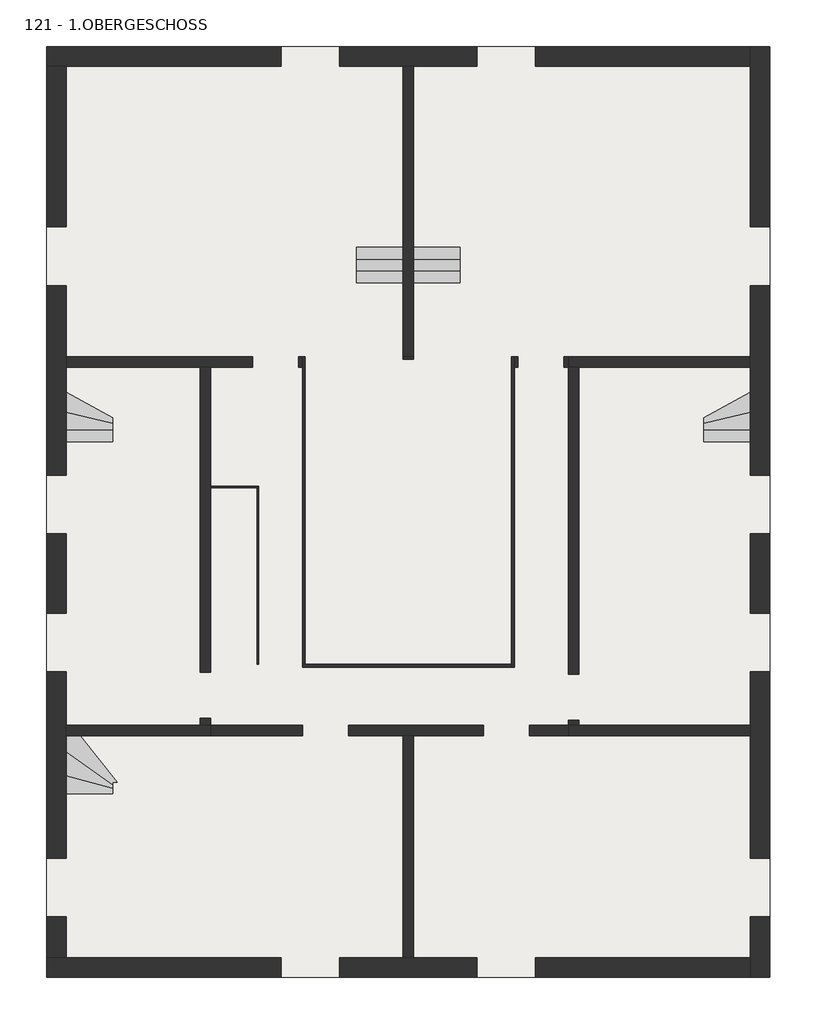
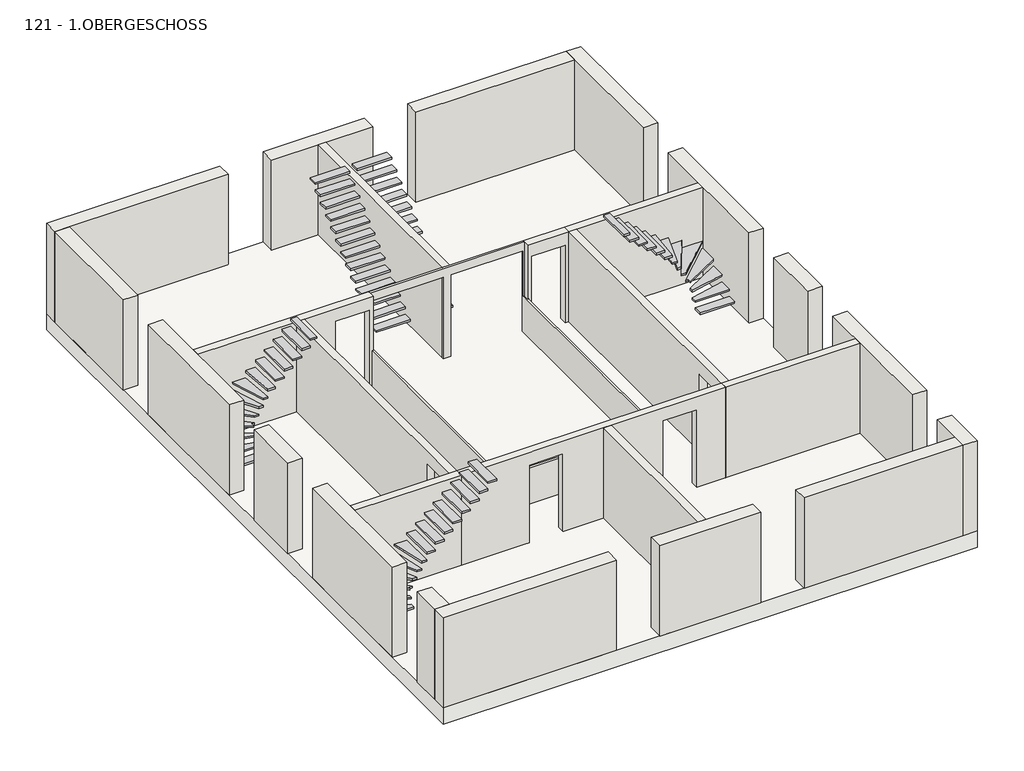
# One storey: 20 walls, 10 stairs, 1 slab.
"""IFC4 building model written with IfcOpenShell, lengths in millimetres."""

import ifcopenshell
import ifcopenshell.guid

model = None  # the IFC model being written
_history = None  # IfcOwnerHistory: only IFC2X3 demands one
_inside = {}  # id of a spatial element -> (the spatial element, [elements in it])
_under = {}  # id of a project, library or spatial element -> (it, [spatial elements below it])
_declared = {}  # id of a project -> (the project, [libraries it declares])
_typed = {}  # id of a type object -> (the type object, [elements of that type])
_made_of = {}  # id of a material, layer set ... -> (it, [elements and type objects made of it])


def new_model(schema):
    """Start an empty IFC model of exactly this schema.

    Asked for "IFC4X3", IfcOpenShell would pick the latest addendum, in which some entities
    have other attributes; the version numbers below select the first issue.
    IFC2X3 requires an IfcOwnerHistory on every rooted entity: one is made here for all.
    """
    global model, _history
    if schema == "IFC4X3":
        model = ifcopenshell.file(schema_version=(4, 3, 0, 0))
    else:
        model = ifcopenshell.file(schema=schema)
    _inside.clear()
    _under.clear()
    _declared.clear()
    _typed.clear()
    _made_of.clear()
    _history = None
    if model.schema == "IFC2X3":
        org = make("IfcOrganization", Name="unknown")
        user = make(
            "IfcPersonAndOrganization",
            ThePerson=make("IfcPerson", FamilyName="unknown"),
            TheOrganization=org,
        )
        app = make(
            "IfcApplication",
            ApplicationDeveloper=org,
            Version="unknown",
            ApplicationFullName="unknown",
            ApplicationIdentifier="unknown",
        )
        _history = make(
            "IfcOwnerHistory",
            OwningUser=user,
            OwningApplication=app,
            ChangeAction="ADDED",
            CreationDate=0,
        )
    return model


def make(cls, **values):
    """One entity of the class cls with the attributes given. An attribute that is None is left unset."""
    return model.create_entity(
        cls, **{name: value for name, value in values.items() if value is not None}
    )


def rooted(cls, **values):
    """An entity with a GlobalId (a new one), such as an element, a storey or a relation."""
    return make(cls, GlobalId=ifcopenshell.guid.new(), OwnerHistory=_history, **values)


def si_unit(unit_type, name, prefix=None):
    """IfcSIUnit, for example si_unit("LENGTHUNIT", "METRE", prefix="MILLI")."""
    return make("IfcSIUnit", UnitType=unit_type, Prefix=prefix, Name=name)


def assignment(units):
    """IfcUnitAssignment: the units of a project."""
    return None if units is None else make("IfcUnitAssignment", Units=units)


def point(xyz):
    """IfcCartesianPoint."""
    return None if xyz is None else make("IfcCartesianPoint", Coordinates=xyz)


def direction(xyz):
    """IfcDirection."""
    return None if xyz is None else make("IfcDirection", DirectionRatios=xyz)


def frame(location, z_axis=None, x_axis=None):
    """IfcAxis2Placement3D, a coordinate frame: its origin and axes. An axis left out is left unset."""
    return make(
        "IfcAxis2Placement3D",
        Location=point(location),
        Axis=direction(z_axis),
        RefDirection=direction(x_axis),
    )


def origin():
    """The frame at (0, 0, 0) with its axes left unset."""
    return frame((0.0, 0.0, 0.0))


def place(relative_to, where):
    """IfcLocalPlacement: puts the frame where relative to a parent placement (None: the world)."""
    return make(
        "IfcLocalPlacement", PlacementRelTo=relative_to, RelativePlacement=where
    )


def context(
    kind, dimensions, precision=None, world=None, true_north=None, identifier=None
):
    """IfcGeometricRepresentationContext, for example the 3D "Model" context."""
    return make(
        "IfcGeometricRepresentationContext",
        ContextIdentifier=identifier,
        ContextType=kind,
        CoordinateSpaceDimension=dimensions,
        Precision=precision,
        WorldCoordinateSystem=world,
        TrueNorth=true_north,
    )


def project(units=None, contexts=None):
    """IfcProject with its units and contexts."""
    return rooted(
        "IfcProject",
        Name="project",
        RepresentationContexts=contexts,
        UnitsInContext=assignment(units),
    )


def spatial(cls, under=None, at=None, **own):
    """A site, building, storey or space (cls), placed at a placement, below another one or the project."""
    s = rooted(cls, ObjectPlacement=at, **own)
    if under is not None:
        _under.setdefault(under.id(), (under, []))[1].append(s)
    return s


def polyline(points):
    """IfcPolyline through the points."""
    return make("IfcPolyline", Points=[point(p) for p in points])


def outline(outer, holes=None, kind="AREA"):
    """IfcArbitraryClosedProfileDef: a profile drawn as a closed curve; with holes, ...WithVoids."""
    if holes is None:
        return make("IfcArbitraryClosedProfileDef", ProfileType=kind, OuterCurve=outer)
    return make(
        "IfcArbitraryProfileDefWithVoids",
        ProfileType=kind,
        OuterCurve=outer,
        InnerCurves=holes,
    )


def extrude(swept, where, along, depth):
    """IfcExtrudedAreaSolid: the profile swept, set in the frame where, extruded along a direction by depth."""
    return make(
        "IfcExtrudedAreaSolid",
        SweptArea=swept,
        Position=where,
        ExtrudedDirection=direction(along),
        Depth=depth,
    )


def faces_of(points, faces, orient=None, outer=None):
    """IfcFace entities. A face is a list of loops; a loop is a list of indices into points, from 0.

    orient and outer hold one flag for each loop. By default every Orientation is true, the
    first loop of a face is its IfcFaceOuterBound and the others are IfcFaceBound.
    """
    made = []
    for i, loops in enumerate(faces):
        bounds = []
        for j, loop in enumerate(loops):
            is_outer = j == 0 if outer is None else outer[i][j]
            bounds.append(
                make(
                    "IfcFaceOuterBound" if is_outer else "IfcFaceBound",
                    Bound=make("IfcPolyLoop", Polygon=[points[k] for k in loop]),
                    Orientation=True if orient is None else orient[i][j],
                )
            )
        made.append(make("IfcFace", Bounds=bounds))
    return made


def faceted_brep(points, faces, orient=None, outer=None, voids=None):
    """IfcFacetedBrep: a solid bounded by flat faces; with voids (closed shells), ...WithVoids."""
    shared = [point(p) for p in points]
    hull = make("IfcClosedShell", CfsFaces=faces_of(shared, faces, orient, outer))
    if voids is None:
        return make("IfcFacetedBrep", Outer=hull)
    return make(
        "IfcFacetedBrepWithVoids",
        Outer=hull,
        Voids=[
            make(cls, CfsFaces=faces_of(shared, fs, o, b)) for cls, fs, o, b in voids
        ],
    )


def shape(context_of_items, identifier, shape_type, items):
    """IfcShapeRepresentation: the items that make up one representation, for example the "Body"."""
    return make(
        "IfcShapeRepresentation",
        ContextOfItems=context_of_items,
        RepresentationIdentifier=identifier,
        RepresentationType=shape_type,
        Items=items,
    )


def source(mapping_origin, context_of_items, identifier, shape_type, items):
    """IfcRepresentationMap: a shape defined once, which mapped items show again and again."""
    return make(
        "IfcRepresentationMap",
        MappingOrigin=mapping_origin,
        MappedRepresentation=shape(context_of_items, identifier, shape_type, items),
    )


def transform(
    local_origin,
    x_axis=None,
    y_axis=None,
    z_axis=None,
    scale=None,
    scale2=None,
    scale3=None,
    uniform=True,
):
    """IfcCartesianTransformationOperator3D, or its non-uniform kind. x_axis, y_axis, z_axis: its Axis1, 2, 3."""
    if uniform:
        return make(
            "IfcCartesianTransformationOperator3D",
            Axis1=direction(x_axis),
            Axis2=direction(y_axis),
            LocalOrigin=point(local_origin),
            Scale=scale,
            Axis3=direction(z_axis),
        )
    return make(
        "IfcCartesianTransformationOperator3DnonUniform",
        Axis1=direction(x_axis),
        Axis2=direction(y_axis),
        LocalOrigin=point(local_origin),
        Scale=scale,
        Axis3=direction(z_axis),
        Scale2=scale2,
        Scale3=scale3,
    )


def mapped(mapping_source, mapping_target):
    """IfcMappedItem: shows the shape of a source again, moved by a transform."""
    return make(
        "IfcMappedItem", MappingSource=mapping_source, MappingTarget=mapping_target
    )


def made_of(thing, what):
    """Note that an element or type object is made of a material, layer set ...; save() writes the relation."""
    if what is not None:
        _made_of.setdefault(what.id(), (what, []))[1].append(thing)
    return thing


def element(
    cls,
    number,
    at=None,
    inside=None,
    cuts=None,
    type_object=None,
    material=None,
    context=None,
    identifier="Body",
    shape_type=None,
    held_by="IfcProductDefinitionShape",
    body=None,
    shapes=None,
    **own,
):
    """One element of the class cls, such as IfcWall. Its Tag is "e" and its number.

    at: its placement. inside: the storey or other place that contains it. cuts: it is an
    opening in that element (IfcRelVoidsElement). A single representation is given by context,
    identifier, shape_type and body (its items); several are given by shapes. held_by: the class
    of the entity that holds the representations. save() writes the other relations.
    """
    e = rooted(cls, Tag="e%d" % number, ObjectPlacement=at, **own)
    if body is not None:
        shapes = [shape(context, identifier, shape_type, body)]
    if shapes is not None:
        e.Representation = make(held_by, Representations=shapes)
    if inside is not None:
        _inside.setdefault(inside.id(), (inside, []))[1].append(e)
    if cuts is not None:
        rooted(
            "IfcRelVoidsElement", RelatingBuildingElement=cuts, RelatedOpeningElement=e
        )
    if type_object is not None:
        _typed.setdefault(type_object.id(), (type_object, []))[1].append(e)
    return made_of(e, material)


def aggregate(whole, parts):
    """IfcRelAggregates: a whole, such as a stair, and the parts it consists of."""
    return rooted("IfcRelAggregates", RelatingObject=whole, RelatedObjects=parts)


def save(model, path):
    """Write the relations noted so far, then the file.

    IfcRelAggregates (storeys below a building ...), IfcRelContainedInSpatialStructure (elements
    in a storey), IfcRelDefinesByType, IfcRelAssociatesMaterial and IfcRelDeclares: one each for
    every whole, place, type object, material and project.
    """
    for whole, parts in _under.values():
        aggregate(whole, parts)
    for where, things in _inside.values():
        rooted(
            "IfcRelContainedInSpatialStructure",
            RelatedElements=things,
            RelatingStructure=where,
        )
    for kind, things in _typed.values():
        rooted("IfcRelDefinesByType", RelatedObjects=things, RelatingType=kind)
    for what, things in _made_of.values():
        rooted("IfcRelAssociatesMaterial", RelatedObjects=things, RelatingMaterial=what)
    for by, libraries in _declared.values():
        rooted("IfcRelDeclares", RelatingContext=by, RelatedDefinitions=libraries)
    model.write(path)


def slab_91406d58(model_context):
    return source(origin(), model_context, "Body", "SweptSolid", [
        extrude(outline(polyline([(15500.0, 19550.0), (15500.0, 1547.1380981), (1500.0, 1547.1380981), (1500.0, 19550.0), (15500.0, 19550.0)])), frame((0.0, 0.0, 2880.0), z_axis=(0.0, 0.0, 1.0), x_axis=(1.0, 0.0, 0.0)), (0.0, 0.0, 1.0), 450.0),
    ])


def stair_92ba3d55(model_context):
    return source(origin(), model_context, "Body", "SweptSolid", [
        extrude(outline(polyline([(160077.7593015, 32139.1812131), (160077.7593015, 32029.7962965), (159177.7593015, 32029.7962965), (159177.7593015, 32381.5903923), (160077.7593015, 32139.1812131)])), frame((0.0, 0.0, 3480.0), z_axis=(0.0, 0.0, 1.0), x_axis=(1.0, 0.0, 0.0)), (0.0, 0.0, 1.0), 50.0),
        extrude(outline(polyline([(160077.7593015, 32208.6851854), (160077.7593015, 32139.1812131), (159177.7593015, 32381.5903923), (159177.7593015, 32851.1265298), (160077.7593015, 32208.6851854)])), frame((0.0, 0.0, 3680.0), z_axis=(0.0, 0.0, 1.0), x_axis=(1.0, 0.0, 0.0)), (0.0, 0.0, 1.0), 50.0),
        extrude(outline(polyline([(159450.38828, 33159.7962965), (160164.4298971, 32259.7962965), (160077.7593015, 32259.7962965), (160077.7593015, 32208.6851854), (159177.7593015, 32851.1265298), (159177.7593015, 33159.7962965), (159450.38828, 33159.7962965)])), frame((0.0, 0.0, 3880.0), z_axis=(0.0, 0.0, 1.0), x_axis=(1.0, 0.0, 0.0)), (0.0, 0.0, 1.0), 50.0),
        extrude(outline(polyline([(160285.4396784, 32259.7962965), (160164.4298971, 32259.7962965), (159450.38828, 33159.7962965), (159877.5404106, 33159.7962965), (160285.4396784, 32259.7962965)])), frame((0.0, 0.0, 4080.0), z_axis=(0.0, 0.0, 1.0), x_axis=(1.0, 0.0, 0.0)), (0.0, 0.0, 1.0), 50.0),
        extrude(outline(polyline([(160412.2916695, 32259.7962965), (160285.4396784, 32259.7962965), (159877.5404106, 33159.7962965), (160212.4306066, 33159.7962965), (160412.2916695, 32259.7962965)])), frame((0.0, 0.0, 4280.0), z_axis=(0.0, 0.0, 1.0), x_axis=(1.0, 0.0, 0.0)), (0.0, 0.0, 1.0), 50.0),
        extrude(outline(polyline([(160546.5910216, 32259.7962965), (160412.2916695, 32259.7962965), (160212.4306066, 33159.7962965), (160538.1312545, 33159.7962965), (160546.5910216, 32259.7962965)])), frame((0.0, 0.0, 4480.0), z_axis=(0.0, 0.0, 1.0), x_axis=(1.0, 0.0, 0.0)), (0.0, 0.0, 1.0), 50.0),
        extrude(outline(polyline([(160772.3611381, 32259.7962965), (160546.5910216, 32259.7962965), (160538.1312545, 33159.7962965), (160772.3611381, 33159.7962965), (160772.3611381, 32259.7962965)])), frame((0.0, 0.0, 4680.0), z_axis=(0.0, 0.0, 1.0), x_axis=(1.0, 0.0, 0.0)), (0.0, 0.0, 1.0), 50.0),
        extrude(outline(polyline([(161002.3611381, 32259.7962965), (160772.3611381, 32259.7962965), (160772.3611381, 33159.7962965), (161002.3611381, 33159.7962965), (161002.3611381, 32259.7962965)])), frame((0.0, 0.0, 4880.0), z_axis=(0.0, 0.0, 1.0), x_axis=(1.0, 0.0, 0.0)), (0.0, 0.0, 1.0), 50.0),
        extrude(outline(polyline([(161232.3611381, 32259.7962965), (161002.3611381, 32259.7962965), (161002.3611381, 33159.7962965), (161232.3611381, 33159.7962965), (161232.3611381, 32259.7962965)])), frame((0.0, 0.0, 5080.0), z_axis=(0.0, 0.0, 1.0), x_axis=(1.0, 0.0, 0.0)), (0.0, 0.0, 1.0), 50.0),
        extrude(outline(polyline([(161462.3611381, 32259.7962965), (161232.3611381, 32259.7962965), (161232.3611381, 33159.7962965), (161462.3611381, 33159.7962965), (161462.3611381, 32259.7962965)])), frame((0.0, 0.0, 5280.0), z_axis=(0.0, 0.0, 1.0), x_axis=(1.0, 0.0, 0.0)), (0.0, 0.0, 1.0), 50.0),
        extrude(outline(polyline([(161692.3611381, 32259.7962965), (161462.3611381, 32259.7962965), (161462.3611381, 33159.7962965), (161692.3611381, 33159.7962965), (161692.3611381, 32259.7962965)])), frame((0.0, 0.0, 5480.0), z_axis=(0.0, 0.0, 1.0), x_axis=(1.0, 0.0, 0.0)), (0.0, 0.0, 1.0), 50.0),
        extrude(outline(polyline([(161922.3611381, 32259.7962965), (161692.3611381, 32259.7962965), (161692.3611381, 33159.7962965), (161922.3611381, 33159.7962965), (161922.3611381, 32259.7962965)])), frame((0.0, 0.0, 5680.0), z_axis=(0.0, 0.0, 1.0), x_axis=(1.0, 0.0, 0.0)), (0.0, 0.0, 1.0), 50.0),
        extrude(outline(polyline([(162152.3611381, 32259.7962965), (161922.3611381, 32259.7962965), (161922.3611381, 33159.7962965), (162152.3611381, 33159.7962965), (162152.3611381, 32259.7962965)])), frame((0.0, 0.0, 5880.0), z_axis=(0.0, 0.0, 1.0), x_axis=(1.0, 0.0, 0.0)), (0.0, 0.0, 1.0), 50.0),
        extrude(outline(polyline([(162382.3611381, 32259.7962965), (162152.3611381, 32259.7962965), (162152.3611381, 33159.7962965), (162382.3611381, 33159.7962965), (162382.3611381, 32259.7962965)])), frame((0.0, 0.0, 6080.0), z_axis=(0.0, 0.0, 1.0), x_axis=(1.0, 0.0, 0.0)), (0.0, 0.0, 1.0), 50.0),
    ])


def stair_5d17669e(model_context):
    return source(origin(), model_context, "Body", "SweptSolid", [
        extrude(outline(polyline([(166797.7593015, 42144.7962965), (166797.7593015, 41914.7962965), (165897.7593015, 41914.7962965), (165897.7593015, 42144.7962965), (166797.7593015, 42144.7962965)])), frame((0.0, 0.0, 3482.1428571), z_axis=(0.0, 0.0, 1.0), x_axis=(1.0, 0.0, 0.0)), (0.0, 0.0, 1.0), 50.0),
        extrude(outline(polyline([(166797.7593015, 42374.7962965), (166797.7593015, 42144.7962965), (165897.7593015, 42144.7962965), (165897.7593015, 42374.7962965), (166797.7593015, 42374.7962965)])), frame((0.0, 0.0, 3684.2857143), z_axis=(0.0, 0.0, 1.0), x_axis=(1.0, 0.0, 0.0)), (0.0, 0.0, 1.0), 50.0),
        extrude(outline(polyline([(166797.7593015, 42604.7962965), (166797.7593015, 42374.7962965), (165897.7593015, 42374.7962965), (165897.7593015, 42604.7962965), (166797.7593015, 42604.7962965)])), frame((0.0, 0.0, 3886.4285714), z_axis=(0.0, 0.0, 1.0), x_axis=(1.0, 0.0, 0.0)), (0.0, 0.0, 1.0), 50.0),
        extrude(outline(polyline([(166797.7593015, 42834.7962965), (166797.7593015, 42604.7962965), (165897.7593015, 42604.7962965), (165897.7593015, 42834.7962965), (166797.7593015, 42834.7962965)])), frame((0.0, 0.0, 4088.5714286), z_axis=(0.0, 0.0, 1.0), x_axis=(1.0, 0.0, 0.0)), (0.0, 0.0, 1.0), 50.0),
        extrude(outline(polyline([(166797.7593015, 43064.7962965), (166797.7593015, 42834.7962965), (165897.7593015, 42834.7962965), (165897.7593015, 43064.7962965), (166797.7593015, 43064.7962965)])), frame((0.0, 0.0, 4290.7142857), z_axis=(0.0, 0.0, 1.0), x_axis=(1.0, 0.0, 0.0)), (0.0, 0.0, 1.0), 50.0),
        extrude(outline(polyline([(166797.7593015, 43294.7962965), (166797.7593015, 43064.7962965), (165897.7593015, 43064.7962965), (165897.7593015, 43294.7962965), (166797.7593015, 43294.7962965)])), frame((0.0, 0.0, 4492.8571429), z_axis=(0.0, 0.0, 1.0), x_axis=(1.0, 0.0, 0.0)), (0.0, 0.0, 1.0), 50.0),
        extrude(outline(polyline([(166797.7593015, 43524.7962965), (166797.7593015, 43294.7962965), (165897.7593015, 43294.7962965), (165897.7593015, 43524.7962965), (166797.7593015, 43524.7962965)])), frame((0.0, 0.0, 4695.0), z_axis=(0.0, 0.0, 1.0), x_axis=(1.0, 0.0, 0.0)), (0.0, 0.0, 1.0), 50.0),
        extrude(outline(polyline([(166797.7593015, 43754.7962965), (166797.7593015, 43524.7962965), (165897.7593015, 43524.7962965), (165897.7593015, 43754.7962965), (166797.7593015, 43754.7962965)])), frame((0.0, 0.0, 4897.1428571), z_axis=(0.0, 0.0, 1.0), x_axis=(1.0, 0.0, 0.0)), (0.0, 0.0, 1.0), 50.0),
        extrude(outline(polyline([(166797.7593015, 43984.7962965), (166797.7593015, 43754.7962965), (165897.7593015, 43754.7962965), (165897.7593015, 43984.7962965), (166797.7593015, 43984.7962965)])), frame((0.0, 0.0, 5099.2857143), z_axis=(0.0, 0.0, 1.0), x_axis=(1.0, 0.0, 0.0)), (0.0, 0.0, 1.0), 50.0),
        extrude(outline(polyline([(166797.7593015, 44214.7962965), (166797.7593015, 43984.7962965), (165897.7593015, 43984.7962965), (165897.7593015, 44214.7962965), (166797.7593015, 44214.7962965)])), frame((0.0, 0.0, 5301.4285714), z_axis=(0.0, 0.0, 1.0), x_axis=(1.0, 0.0, 0.0)), (0.0, 0.0, 1.0), 50.0),
        extrude(outline(polyline([(166797.7593015, 44444.7962965), (166797.7593015, 44214.7962965), (165897.7593015, 44214.7962965), (165897.7593015, 44444.7962965), (166797.7593015, 44444.7962965)])), frame((0.0, 0.0, 5503.5714286), z_axis=(0.0, 0.0, 1.0), x_axis=(1.0, 0.0, 0.0)), (0.0, 0.0, 1.0), 50.0),
        extrude(outline(polyline([(166797.7593015, 44674.7962965), (166797.7593015, 44444.7962965), (165897.7593015, 44444.7962965), (165897.7593015, 44674.7962965), (166797.7593015, 44674.7962965)])), frame((0.0, 0.0, 5705.7142857), z_axis=(0.0, 0.0, 1.0), x_axis=(1.0, 0.0, 0.0)), (0.0, 0.0, 1.0), 50.0),
        extrude(outline(polyline([(166797.7593015, 44904.7962965), (166797.7593015, 44674.7962965), (165897.7593015, 44674.7962965), (165897.7593015, 44904.7962965), (166797.7593015, 44904.7962965)])), frame((0.0, 0.0, 5907.8571429), z_axis=(0.0, 0.0, 1.0), x_axis=(1.0, 0.0, 0.0)), (0.0, 0.0, 1.0), 50.0),
    ])


def stair_42ef58a3(model_context):
    return source(origin(), model_context, "Body", "SweptSolid", [
        extrude(outline(polyline([(165697.7593015, 42144.7962965), (165697.7593015, 41914.7962965), (164797.7593015, 41914.7962965), (164797.7593015, 42144.7962965), (165697.7593015, 42144.7962965)])), frame((0.0, 0.0, 3482.1428571), z_axis=(0.0, 0.0, 1.0), x_axis=(1.0, 0.0, 0.0)), (0.0, 0.0, 1.0), 50.0),
        extrude(outline(polyline([(165697.7593015, 42374.7962965), (165697.7593015, 42144.7962965), (164797.7593015, 42144.7962965), (164797.7593015, 42374.7962965), (165697.7593015, 42374.7962965)])), frame((0.0, 0.0, 3684.2857143), z_axis=(0.0, 0.0, 1.0), x_axis=(1.0, 0.0, 0.0)), (0.0, 0.0, 1.0), 50.0),
        extrude(outline(polyline([(165697.7593015, 42604.7962965), (165697.7593015, 42374.7962965), (164797.7593015, 42374.7962965), (164797.7593015, 42604.7962965), (165697.7593015, 42604.7962965)])), frame((0.0, 0.0, 3886.4285714), z_axis=(0.0, 0.0, 1.0), x_axis=(1.0, 0.0, 0.0)), (0.0, 0.0, 1.0), 50.0),
        extrude(outline(polyline([(165697.7593015, 42834.7962965), (165697.7593015, 42604.7962965), (164797.7593015, 42604.7962965), (164797.7593015, 42834.7962965), (165697.7593015, 42834.7962965)])), frame((0.0, 0.0, 4088.5714286), z_axis=(0.0, 0.0, 1.0), x_axis=(1.0, 0.0, 0.0)), (0.0, 0.0, 1.0), 50.0),
        extrude(outline(polyline([(165697.7593015, 43064.7962965), (165697.7593015, 42834.7962965), (164797.7593015, 42834.7962965), (164797.7593015, 43064.7962965), (165697.7593015, 43064.7962965)])), frame((0.0, 0.0, 4290.7142857), z_axis=(0.0, 0.0, 1.0), x_axis=(1.0, 0.0, 0.0)), (0.0, 0.0, 1.0), 50.0),
        extrude(outline(polyline([(165697.7593015, 43294.7962965), (165697.7593015, 43064.7962965), (164797.7593015, 43064.7962965), (164797.7593015, 43294.7962965), (165697.7593015, 43294.7962965)])), frame((0.0, 0.0, 4492.8571429), z_axis=(0.0, 0.0, 1.0), x_axis=(1.0, 0.0, 0.0)), (0.0, 0.0, 1.0), 50.0),
        extrude(outline(polyline([(165697.7593015, 43524.7962965), (165697.7593015, 43294.7962965), (164797.7593015, 43294.7962965), (164797.7593015, 43524.7962965), (165697.7593015, 43524.7962965)])), frame((0.0, 0.0, 4695.0), z_axis=(0.0, 0.0, 1.0), x_axis=(1.0, 0.0, 0.0)), (0.0, 0.0, 1.0), 50.0),
        extrude(outline(polyline([(165697.7593015, 43754.7962965), (165697.7593015, 43524.7962965), (164797.7593015, 43524.7962965), (164797.7593015, 43754.7962965), (165697.7593015, 43754.7962965)])), frame((0.0, 0.0, 4897.1428571), z_axis=(0.0, 0.0, 1.0), x_axis=(1.0, 0.0, 0.0)), (0.0, 0.0, 1.0), 50.0),
        extrude(outline(polyline([(165697.7593015, 43984.7962965), (165697.7593015, 43754.7962965), (164797.7593015, 43754.7962965), (164797.7593015, 43984.7962965), (165697.7593015, 43984.7962965)])), frame((0.0, 0.0, 5099.2857143), z_axis=(0.0, 0.0, 1.0), x_axis=(1.0, 0.0, 0.0)), (0.0, 0.0, 1.0), 50.0),
        extrude(outline(polyline([(165697.7593015, 44214.7962965), (165697.7593015, 43984.7962965), (164797.7593015, 43984.7962965), (164797.7593015, 44214.7962965), (165697.7593015, 44214.7962965)])), frame((0.0, 0.0, 5301.4285714), z_axis=(0.0, 0.0, 1.0), x_axis=(1.0, 0.0, 0.0)), (0.0, 0.0, 1.0), 50.0),
        extrude(outline(polyline([(165697.7593015, 44444.7962965), (165697.7593015, 44214.7962965), (164797.7593015, 44214.7962965), (164797.7593015, 44444.7962965), (165697.7593015, 44444.7962965)])), frame((0.0, 0.0, 5503.5714286), z_axis=(0.0, 0.0, 1.0), x_axis=(1.0, 0.0, 0.0)), (0.0, 0.0, 1.0), 50.0),
        extrude(outline(polyline([(165697.7593015, 44674.7962965), (165697.7593015, 44444.7962965), (164797.7593015, 44444.7962965), (164797.7593015, 44674.7962965), (165697.7593015, 44674.7962965)])), frame((0.0, 0.0, 5705.7142857), z_axis=(0.0, 0.0, 1.0), x_axis=(1.0, 0.0, 0.0)), (0.0, 0.0, 1.0), 50.0),
        extrude(outline(polyline([(165697.7593015, 44904.7962965), (165697.7593015, 44674.7962965), (164797.7593015, 44674.7962965), (164797.7593015, 44904.7962965), (165697.7593015, 44904.7962965)])), frame((0.0, 0.0, 5907.8571429), z_axis=(0.0, 0.0, 1.0), x_axis=(1.0, 0.0, 0.0)), (0.0, 0.0, 1.0), 50.0),
    ])


def stair_4856ba97(model_context):
    return source(origin(), model_context, "Body", "SweptSolid", [
        extrude(outline(polyline([(159177.7593015, 39074.7962965), (160077.7593015, 39074.7962965), (160077.7593015, 38844.7962965), (159177.7593015, 38844.7962965), (159177.7593015, 39074.7962965)])), frame((0.0, 0.0, 3482.1428571), z_axis=(0.0, 0.0, 1.0), x_axis=(1.0, 0.0, 0.0)), (0.0, 0.0, 1.0), 50.0),
        extrude(outline(polyline([(159177.7593015, 39407.7634868), (160077.7593015, 39201.8291061), (160077.7593015, 39074.7962965), (159177.7593015, 39074.7962965), (159177.7593015, 39407.7634868)])), frame((0.0, 0.0, 3684.2857143), z_axis=(0.0, 0.0, 1.0), x_axis=(1.0, 0.0, 0.0)), (0.0, 0.0, 1.0), 50.0),
        extrude(outline(polyline([(159177.7593015, 39801.0914939), (160077.7593015, 39301.7193734), (160077.7593015, 39201.8291061), (159177.7593015, 39407.7634868), (159177.7593015, 39801.0914939)])), frame((0.0, 0.0, 3886.4285714), z_axis=(0.0, 0.0, 1.0), x_axis=(1.0, 0.0, 0.0)), (0.0, 0.0, 1.0), 50.0),
        extrude(outline(polyline([(159177.7593015, 40284.7962965), (159200.4297176, 40284.7962965), (160147.7593015, 39384.7962965), (160077.7593015, 39384.7962965), (160077.7593015, 39301.7193734), (159177.7593015, 39801.0914939), (159177.7593015, 40284.7962965)])), frame((0.0, 0.0, 4088.5714286), z_axis=(0.0, 0.0, 1.0), x_axis=(1.0, 0.0, 0.0)), (0.0, 0.0, 1.0), 50.0),
        extrude(outline(polyline([(159730.1980238, 40284.7962965), (160258.7713888, 39384.7962965), (160147.7593015, 39384.7962965), (159200.4297176, 40284.7962965), (159730.1980238, 40284.7962965)])), frame((0.0, 0.0, 4290.7142857), z_axis=(0.0, 0.0, 1.0), x_axis=(1.0, 0.0, 0.0)), (0.0, 0.0, 1.0), 50.0),
        extrude(outline(polyline([(160089.4284981, 40284.7962965), (160375.293778, 39384.7962965), (160258.7713888, 39384.7962965), (159730.1980238, 40284.7962965), (160089.4284981, 40284.7962965)])), frame((0.0, 0.0, 4492.8571429), z_axis=(0.0, 0.0, 1.0), x_axis=(1.0, 0.0, 0.0)), (0.0, 0.0, 1.0), 50.0),
        extrude(outline(polyline([(160425.6183342, 40284.7962965), (160499.1039419, 39384.7962965), (160375.293778, 39384.7962965), (160089.4284981, 40284.7962965), (160425.6183342, 40284.7962965)])), frame((0.0, 0.0, 4695.0), z_axis=(0.0, 0.0, 1.0), x_axis=(1.0, 0.0, 0.0)), (0.0, 0.0, 1.0), 50.0),
        extrude(outline(polyline([(160692.3611381, 40284.7962965), (160692.3611381, 39384.7962965), (160499.1039419, 39384.7962965), (160425.6183342, 40284.7962965), (160692.3611381, 40284.7962965)])), frame((0.0, 0.0, 4897.1428571), z_axis=(0.0, 0.0, 1.0), x_axis=(1.0, 0.0, 0.0)), (0.0, 0.0, 1.0), 50.0),
        extrude(outline(polyline([(160922.3611381, 40284.7962965), (160922.3611381, 39384.7962965), (160692.3611381, 39384.7962965), (160692.3611381, 40284.7962965), (160922.3611381, 40284.7962965)])), frame((0.0, 0.0, 5099.2857143), z_axis=(0.0, 0.0, 1.0), x_axis=(1.0, 0.0, 0.0)), (0.0, 0.0, 1.0), 50.0),
        extrude(outline(polyline([(161152.3611381, 40284.7962965), (161152.3611381, 39384.7962965), (160922.3611381, 39384.7962965), (160922.3611381, 40284.7962965), (161152.3611381, 40284.7962965)])), frame((0.0, 0.0, 5301.4285714), z_axis=(0.0, 0.0, 1.0), x_axis=(1.0, 0.0, 0.0)), (0.0, 0.0, 1.0), 50.0),
        extrude(outline(polyline([(161382.3611381, 40284.7962965), (161382.3611381, 39384.7962965), (161152.3611381, 39384.7962965), (161152.3611381, 40284.7962965), (161382.3611381, 40284.7962965)])), frame((0.0, 0.0, 5503.5714286), z_axis=(0.0, 0.0, 1.0), x_axis=(1.0, 0.0, 0.0)), (0.0, 0.0, 1.0), 50.0),
        extrude(outline(polyline([(161612.3611381, 40284.7962965), (161612.3611381, 39384.7962965), (161382.3611381, 39384.7962965), (161382.3611381, 40284.7962965), (161612.3611381, 40284.7962965)])), frame((0.0, 0.0, 5705.7142857), z_axis=(0.0, 0.0, 1.0), x_axis=(1.0, 0.0, 0.0)), (0.0, 0.0, 1.0), 50.0),
        extrude(outline(polyline([(161772.7593015, 40284.7962965), (161772.7593015, 39384.7962965), (161612.3611381, 39384.7962965), (161612.3611381, 40284.7962965), (161772.7593015, 40284.7962965)])), frame((0.0, 0.0, 5907.8571429), z_axis=(0.0, 0.0, 1.0), x_axis=(1.0, 0.0, 0.0)), (0.0, 0.0, 1.0), 50.0),
    ])


def stair_6893023c(model_context):
    return source(origin(), model_context, "Body", "SweptSolid", [
        extrude(outline(polyline([(171517.7593015, 39074.7962965), (172417.7593015, 39074.7962965), (172417.7593015, 38844.7962965), (171517.7593015, 38844.7962965), (171517.7593015, 39074.7962965)])), frame((0.0, 0.0, 3482.1428571), z_axis=(0.0, 0.0, 1.0), x_axis=(1.0, 0.0, 0.0)), (0.0, 0.0, 1.0), 50.0),
        extrude(outline(polyline([(171517.7593015, 39201.8291061), (172417.7593015, 39407.7634868), (172417.7593015, 39074.7962965), (171517.7593015, 39074.7962965), (171517.7593015, 39201.8291061)])), frame((0.0, 0.0, 3684.2857143), z_axis=(0.0, 0.0, 1.0), x_axis=(1.0, 0.0, 0.0)), (0.0, 0.0, 1.0), 50.0),
        extrude(outline(polyline([(171517.7593015, 39301.7193734), (172417.7593015, 39801.0914939), (172417.7593015, 39407.7634868), (171517.7593015, 39201.8291061), (171517.7593015, 39301.7193734)])), frame((0.0, 0.0, 3886.4285714), z_axis=(0.0, 0.0, 1.0), x_axis=(1.0, 0.0, 0.0)), (0.0, 0.0, 1.0), 50.0),
        extrude(outline(polyline([(171517.7593015, 39384.7962965), (171447.7593015, 39384.7962965), (172395.0888853, 40284.7962965), (172417.7593015, 40284.7962965), (172417.7593015, 39801.0914939), (171517.7593015, 39301.7193734), (171517.7593015, 39384.7962965)])), frame((0.0, 0.0, 4088.5714286), z_axis=(0.0, 0.0, 1.0), x_axis=(1.0, 0.0, 0.0)), (0.0, 0.0, 1.0), 50.0),
        extrude(outline(polyline([(171336.7472141, 39384.7962965), (171865.3205791, 40284.7962965), (172395.0888853, 40284.7962965), (171447.7593015, 39384.7962965), (171336.7472141, 39384.7962965)])), frame((0.0, 0.0, 4290.7142857), z_axis=(0.0, 0.0, 1.0), x_axis=(1.0, 0.0, 0.0)), (0.0, 0.0, 1.0), 50.0),
        extrude(outline(polyline([(171220.2248249, 39384.7962965), (171506.0901048, 40284.7962965), (171865.3205791, 40284.7962965), (171336.7472141, 39384.7962965), (171220.2248249, 39384.7962965)])), frame((0.0, 0.0, 4492.8571429), z_axis=(0.0, 0.0, 1.0), x_axis=(1.0, 0.0, 0.0)), (0.0, 0.0, 1.0), 50.0),
        extrude(outline(polyline([(171096.414661, 39384.7962965), (171169.9002687, 40284.7962965), (171506.0901048, 40284.7962965), (171220.2248249, 39384.7962965), (171096.414661, 39384.7962965)])), frame((0.0, 0.0, 4695.0), z_axis=(0.0, 0.0, 1.0), x_axis=(1.0, 0.0, 0.0)), (0.0, 0.0, 1.0), 50.0),
        extrude(outline(polyline([(170903.1574649, 39384.7962965), (170903.1574649, 40284.7962965), (171169.9002687, 40284.7962965), (171096.414661, 39384.7962965), (170903.1574649, 39384.7962965)])), frame((0.0, 0.0, 4897.1428571), z_axis=(0.0, 0.0, 1.0), x_axis=(1.0, 0.0, 0.0)), (0.0, 0.0, 1.0), 50.0),
        extrude(outline(polyline([(170673.1574649, 39384.7962965), (170673.1574649, 40284.7962965), (170903.1574649, 40284.7962965), (170903.1574649, 39384.7962965), (170673.1574649, 39384.7962965)])), frame((0.0, 0.0, 5099.2857143), z_axis=(0.0, 0.0, 1.0), x_axis=(1.0, 0.0, 0.0)), (0.0, 0.0, 1.0), 50.0),
        extrude(outline(polyline([(170443.1574649, 39384.7962965), (170443.1574649, 40284.7962965), (170673.1574649, 40284.7962965), (170673.1574649, 39384.7962965), (170443.1574649, 39384.7962965)])), frame((0.0, 0.0, 5301.4285714), z_axis=(0.0, 0.0, 1.0), x_axis=(1.0, 0.0, 0.0)), (0.0, 0.0, 1.0), 50.0),
        extrude(outline(polyline([(170213.1574649, 39384.7962965), (170213.1574649, 40284.7962965), (170443.1574649, 40284.7962965), (170443.1574649, 39384.7962965), (170213.1574649, 39384.7962965)])), frame((0.0, 0.0, 5503.5714286), z_axis=(0.0, 0.0, 1.0), x_axis=(1.0, 0.0, 0.0)), (0.0, 0.0, 1.0), 50.0),
        extrude(outline(polyline([(169983.1574649, 39384.7962965), (169983.1574649, 40284.7962965), (170213.1574649, 40284.7962965), (170213.1574649, 39384.7962965), (169983.1574649, 39384.7962965)])), frame((0.0, 0.0, 5705.7142857), z_axis=(0.0, 0.0, 1.0), x_axis=(1.0, 0.0, 0.0)), (0.0, 0.0, 1.0), 50.0),
        extrude(outline(polyline([(169822.7593015, 39384.7962965), (169822.7593015, 40284.7962965), (169983.1574649, 40284.7962965), (169983.1574649, 39384.7962965), (169822.7593015, 39384.7962965)])), frame((0.0, 0.0, 5907.8571429), z_axis=(0.0, 0.0, 1.0), x_axis=(1.0, 0.0, 0.0)), (0.0, 0.0, 1.0), 50.0),
    ])


model = new_model("IFC4")

# Units and contexts
model_context = context("Model", 3, world=origin())
ifc_project = project(units=[si_unit("LENGTHUNIT", "METRE", prefix="MILLI")], contexts=[model_context])

# Site, building, storey
site = spatial("IfcSite", under=ifc_project)
building = spatial("IfcBuilding", under=site)
storey = spatial("IfcBuildingStorey", under=building, Name="121 - 1.OBERGESCHOSS", Elevation=2825.0)

# Slab
placement = place(None, origin())
slab_shape = slab_91406d58(model_context)
element("IfcSlab", 1, ObjectType="Holzdecke 176 : Holzdecke 176", at=placement, inside=storey, context=model_context, shape_type="MappedRepresentation", body=[
    mapped(slab_shape, transform((0.0, 0.0, 0.0), x_axis=(1.0, 0.0, 0.0), y_axis=(0.0, 1.0, 0.0), z_axis=(0.0, 0.0, 1.0))),
])

# Stairs
stair_shape = stair_92ba3d55(model_context)
element("IfcStair", 2, ObjectType="  97010 :   97010", at=placement, inside=storey, context=model_context, shape_type="MappedRepresentation", body=[
    mapped(stair_shape, transform((-157297.7593015, -26934.7962965, 0.0), x_axis=(1.0, 0.0, 0.0), y_axis=(0.0, 1.0, 0.0), z_axis=(0.0, 0.0, 1.0))),
])
stair_2_shape = stair_5d17669e(model_context)
element("IfcStair", 3, ObjectType="  97882 :   97882", at=placement, inside=storey, context=model_context, shape_type="MappedRepresentation", body=[
    mapped(stair_2_shape, transform((-157297.7593015, -26934.7962965, 0.0), x_axis=(1.0, 0.0, 0.0), y_axis=(0.0, 1.0, 0.0), z_axis=(0.0, 0.0, 1.0))),
])
stair_3_shape = stair_42ef58a3(model_context)
element("IfcStair", 4, ObjectType="  98300 :   98300", at=placement, inside=storey, context=model_context, shape_type="MappedRepresentation", body=[
    mapped(stair_3_shape, transform((-157297.7593015, -26934.7962965, 0.0), x_axis=(1.0, 0.0, 0.0), y_axis=(0.0, 1.0, 0.0), z_axis=(0.0, 0.0, 1.0))),
])
stair_4_shape = stair_4856ba97(model_context)
element("IfcStair", 5, ObjectType="  98728 :   98728", at=placement, inside=storey, context=model_context, shape_type="MappedRepresentation", body=[
    mapped(stair_4_shape, transform((-157297.7593015, -26934.7962965, 0.0), x_axis=(1.0, 0.0, 0.0), y_axis=(0.0, 1.0, 0.0), z_axis=(0.0, 0.0, 1.0))),
])
stair_5_shape = stair_6893023c(model_context)
element("IfcStair", 6, ObjectType="  99154 :   99154", at=placement, inside=storey, context=model_context, shape_type="MappedRepresentation", body=[
    mapped(stair_5_shape, transform((-157297.7593015, -26934.7962965, 0.0), x_axis=(1.0, 0.0, 0.0), y_axis=(0.0, 1.0, 0.0), z_axis=(0.0, 0.0, 1.0))),
])
element("IfcStair", 7, ObjectType="  149542 :   149542", at=placement, inside=storey, context=model_context, shape_type="MappedRepresentation", body=[
    mapped(stair_shape, transform((-157297.7593015, -26934.7962965, 0.0), x_axis=(1.0, 0.0, 0.0), y_axis=(0.0, 1.0, 0.0), z_axis=(0.0, 0.0, 1.0))),
])
element("IfcStair", 8, ObjectType="  150414 :   150414", at=placement, inside=storey, context=model_context, shape_type="MappedRepresentation", body=[
    mapped(stair_2_shape, transform((-157297.7593015, -26934.7962965, 0.0), x_axis=(1.0, 0.0, 0.0), y_axis=(0.0, 1.0, 0.0), z_axis=(0.0, 0.0, 1.0))),
])
element("IfcStair", 9, ObjectType="  150832 :   150832", at=placement, inside=storey, context=model_context, shape_type="MappedRepresentation", body=[
    mapped(stair_3_shape, transform((-157297.7593015, -26934.7962965, 0.0), x_axis=(1.0, 0.0, 0.0), y_axis=(0.0, 1.0, 0.0), z_axis=(0.0, 0.0, 1.0))),
])
element("IfcStair", 10, ObjectType="  151260 :   151260", at=placement, inside=storey, context=model_context, shape_type="MappedRepresentation", body=[
    mapped(stair_4_shape, transform((-157297.7593015, -26934.7962965, 0.0), x_axis=(1.0, 0.0, 0.0), y_axis=(0.0, 1.0, 0.0), z_axis=(0.0, 0.0, 1.0))),
])
element("IfcStair", 11, ObjectType="  151686 :   151686", at=placement, inside=storey, context=model_context, shape_type="MappedRepresentation", body=[
    mapped(stair_5_shape, transform((-157297.7593015, -26934.7962965, 0.0), x_axis=(1.0, 0.0, 0.0), y_axis=(0.0, 1.0, 0.0), z_axis=(0.0, 0.0, 1.0))),
])

# Walls
element("IfcWall", 12, ObjectType=" :1166", at=placement, inside=storey, context=model_context, shape_type="SweptSolid", body=[
    extrude(outline(polyline([(5830.0, 10525.0), (5830.0, 6475.0), (4330.0, 6475.0), (4330.0, 6500.0), (5590.0, 6500.0), (5590.0, 8400.0), (3330.0, 8400.0), (3330.0, 8600.0), (5590.0, 8600.0), (5590.0, 10500.0), (4330.0, 10500.0), (4330.0, 10525.0), (5830.0, 10525.0)])), frame((0.0, 13500.0, 0.0), z_axis=(0.0, 1.0, 0.0), x_axis=(0.0, 0.0, 1.0)), (0.0, 0.0, 1.0), 50.0),
])
element("IfcWall", 13, ObjectType="Holzwand:1150", at=placement, inside=storey, context=model_context, shape_type="Brep", body=[
    faceted_brep([(11600.0, 13350.0, 3330.0), (11800.0, 13350.0, 3330.0), (15120.0, 13350.0, 3330.0), (15120.0, 13350.0, 5830.0), (11800.0, 13350.0, 5830.0), (11600.0, 13350.0, 5830.0), (11600.0, 13550.0, 3330.0), (11600.0, 13550.0, 5830.0), (15120.0, 13550.0, 5830.0), (15120.0, 13550.0, 3330.0)], [[[0, 1, 2, 3, 4, 5]], [[6, 7, 8, 9]], [[2, 1, 0, 6, 9]], [[5, 4, 3, 8, 7]], [[0, 5, 7, 6]], [[3, 2, 9, 8]]]),
])
element("IfcWall", 14, ObjectType="Holzwand:1151", at=placement, inside=storey, context=model_context, shape_type="Brep", body=[
    faceted_brep([(4675.0, 6425.0, 3330.0), (4475.0, 6425.0, 3330.0), (1880.0, 6425.0, 3330.0), (1880.0, 6425.0, 5830.0), (4475.0, 6425.0, 5830.0), (4675.0, 6425.0, 5830.0), (4675.0, 6225.0, 3330.0), (4675.0, 6225.0, 5830.0), (1880.0, 6225.0, 5830.0), (1880.0, 6225.0, 3330.0)], [[[0, 1, 2, 3, 4, 5]], [[6, 7, 8, 9]], [[2, 1, 0, 6, 9]], [[5, 4, 3, 8, 7]], [[0, 5, 7, 6]], [[3, 2, 9, 8]]]),
])
element("IfcWall", 15, ObjectType="Holzwand:1153", at=placement, inside=storey, context=model_context, shape_type="Brep", body=[
    faceted_brep([(15120.0, 6425.0, 3330.0), (11800.0, 6425.0, 3330.0), (11600.0, 6425.0, 3330.0), (11600.0, 6425.0, 5830.0), (11800.0, 6425.0, 5830.0), (15120.0, 6425.0, 5830.0), (15120.0, 6225.0, 3330.0), (15120.0, 6225.0, 5830.0), (11600.0, 6225.0, 5830.0), (11600.0, 6225.0, 3330.0)], [[[0, 1, 2, 3, 4, 5]], [[6, 7, 8, 9]], [[2, 1, 0, 6, 9]], [[5, 4, 3, 8, 7]], [[3, 2, 9, 8]], [[0, 5, 7, 6]]]),
])
element("IfcWall", 16, ObjectType="Holzwand:1154", at=placement, inside=storey, context=model_context, shape_type="Brep", body=[
    faceted_brep([(5605.0, 11050.0, 3330.0), (4675.0, 11050.0, 3330.0), (4675.0, 11050.0, 4330.0), (5605.0, 11050.0, 4330.0), (5605.0, 11020.0, 3330.0), (5605.0, 11020.0, 4330.0), (5575.0, 11020.0, 4330.0), (4675.0, 11020.0, 4330.0), (4675.0, 11020.0, 3330.0), (5575.0, 11020.0, 3330.0)], [[[0, 1, 2, 3]], [[4, 5, 6, 7, 8, 9]], [[1, 0, 4, 9, 8]], [[3, 2, 7, 6, 5]], [[0, 3, 5, 4]], [[2, 1, 8, 7]]]),
])
element("IfcWall", 17, ObjectType="Holzwand:1155", at=placement, inside=storey, context=model_context, shape_type="SweptSolid", body=[
    extrude(outline(polyline([(5605.0, 11020.0), (5605.0, 7600.0), (5575.0, 7600.0), (5575.0, 11020.0), (5605.0, 11020.0)])), frame((0.0, 0.0, 3330.0), z_axis=(0.0, 0.0, 1.0), x_axis=(1.0, 0.0, 0.0)), (0.0, 0.0, 1.0), 1000.0),
])
element("IfcWall", 18, ObjectType="Holzwand:1156", at=placement, inside=storey, context=model_context, shape_type="SweptSolid", body=[
    extrude(outline(polyline([(6425.0, 5830.0), (13350.0, 5830.0), (13350.0, 3330.0), (7409.5766702, 3330.0), (7409.5766702, 5480.0), (6524.5766702, 5480.0), (6524.5766702, 3330.0), (6425.0, 3330.0), (6425.0, 5830.0)])), frame((11600.0, 0.0, 0.0), z_axis=(1.0, 0.0, 0.0), x_axis=(0.0, 1.0, 0.0)), (0.0, 0.0, 1.0), 200.0),
])
element("IfcWall", 19, ObjectType="Holzwand:1157", at=placement, inside=storey, context=model_context, shape_type="SweptSolid", body=[
    extrude(outline(polyline([(8600.0, 19170.0), (8600.0, 13550.0), (8400.0, 13550.0), (8400.0, 19170.0), (8600.0, 19170.0)])), frame((0.0, 0.0, 3330.0), z_axis=(0.0, 0.0, 1.0), x_axis=(1.0, 0.0, 0.0)), (0.0, 0.0, 1.0), 2500.0),
])
element("IfcWall", 20, ObjectType="Holzwand:1158", at=placement, inside=storey, context=model_context, shape_type="Brep", body=[
    faceted_brep([(4475.0, 6425.0, 5830.0), (4475.0, 13350.0, 5830.0), (4475.0, 13350.0, 3330.0), (4475.0, 7448.3297038, 3330.0), (4475.0, 7448.3297038, 5480.0), (4475.0, 6563.3297038, 5480.0), (4475.0, 6563.3297038, 3330.0), (4475.0, 6425.0, 3330.0), (4675.0, 13350.0, 5830.0), (4675.0, 6425.0, 5830.0), (4675.0, 6425.0, 3330.0), (4675.0, 6563.3297038, 3330.0), (4675.0, 6563.3297038, 5480.0), (4675.0, 7448.3297038, 5480.0), (4675.0, 7448.3297038, 3330.0), (4675.0, 11020.0, 3330.0), (4675.0, 11050.0, 3330.0), (4675.0, 13350.0, 3330.0)], [[[0, 1, 2, 3, 4, 5, 6, 7]], [[8, 9, 10, 11, 12, 13, 14, 15, 16, 17]], [[2, 17, 16, 15, 14, 3]], [[10, 7, 6, 11]], [[1, 0, 9, 8]], [[5, 12, 11, 6]], [[12, 5, 4, 13]], [[13, 4, 3, 14]], [[0, 7, 10, 9]], [[2, 1, 8, 17]]]),
])
element("IfcWall", 21, ObjectType="Holzwand:1159", at=placement, inside=storey, context=model_context, shape_type="Brep", body=[
    faceted_brep([(11600.0, 6225.0, 5830.0), (8600.0, 6225.0, 5830.0), (8400.0, 6225.0, 5830.0), (4675.0, 6225.0, 5830.0), (4675.0, 6225.0, 3330.0), (6455.0, 6225.0, 3330.0), (6455.0, 6225.0, 5480.0), (7340.0, 6225.0, 5480.0), (7340.0, 6225.0, 3330.0), (8400.0, 6225.0, 3330.0), (8600.0, 6225.0, 3330.0), (9960.0, 6225.0, 3330.0), (9960.0, 6225.0, 5480.0), (10845.0, 6225.0, 5480.0), (10845.0, 6225.0, 3330.0), (11600.0, 6225.0, 3330.0), (4675.0, 6425.0, 5830.0), (11600.0, 6425.0, 5830.0), (11600.0, 6425.0, 3330.0), (10845.0, 6425.0, 3330.0), (10845.0, 6425.0, 5480.0), (9960.0, 6425.0, 5480.0), (9960.0, 6425.0, 3330.0), (7340.0, 6425.0, 3330.0), (7340.0, 6425.0, 5480.0), (6455.0, 6425.0, 5480.0), (6455.0, 6425.0, 3330.0), (4675.0, 6425.0, 3330.0)], [[[0, 1, 2, 3, 4, 5, 6, 7, 8, 9, 10, 11, 12, 13, 14, 15]], [[16, 17, 18, 19, 20, 21, 22, 23, 24, 25, 26, 27]], [[15, 14, 19, 18]], [[22, 11, 10, 9, 8, 23]], [[4, 27, 26, 5]], [[3, 2, 1, 0, 17, 16]], [[13, 20, 19, 14]], [[20, 13, 12, 21]], [[21, 12, 11, 22]], [[7, 24, 23, 8]], [[24, 7, 6, 25]], [[25, 6, 5, 26]], [[0, 15, 18, 17]], [[4, 3, 16, 27]]]),
])
element("IfcWall", 22, ObjectType="Holzwand:1160", at=placement, inside=storey, context=model_context, shape_type="SweptSolid", body=[
    extrude(outline(polyline([(8600.0, 6225.0), (8600.0, 1927.1380981), (8400.0, 1927.1380981), (8400.0, 6225.0), (8600.0, 6225.0)])), frame((0.0, 0.0, 3330.0), z_axis=(0.0, 0.0, 1.0), x_axis=(1.0, 0.0, 0.0)), (0.0, 0.0, 1.0), 2500.0),
])
element("IfcWall", 23, ObjectType="Holzwand:1162", at=placement, inside=storey, context=model_context, shape_type="Brep", body=[
    faceted_brep([(6475.0, 13350.0, 5830.0), (4675.0, 13350.0, 5830.0), (4475.0, 13350.0, 5830.0), (1880.0, 13350.0, 5830.0), (1880.0, 13350.0, 3330.0), (4475.0, 13350.0, 3330.0), (4675.0, 13350.0, 3330.0), (5490.0, 13350.0, 3330.0), (5490.0, 13350.0, 5480.0), (6375.0, 13350.0, 5480.0), (6375.0, 13350.0, 3330.0), (6450.0, 13350.0, 3330.0), (6450.0, 13350.0, 4330.0), (6475.0, 13350.0, 4330.0), (1880.0, 13550.0, 5830.0), (6475.0, 13550.0, 5830.0), (6475.0, 13550.0, 4330.0), (6450.0, 13550.0, 4330.0), (6450.0, 13550.0, 3330.0), (6375.0, 13550.0, 3330.0), (6375.0, 13550.0, 5480.0), (5490.0, 13550.0, 5480.0), (5490.0, 13550.0, 3330.0), (1880.0, 13550.0, 3330.0)], [[[0, 1, 2, 3, 4, 5, 6, 7, 8, 9, 10, 11, 12, 13]], [[14, 15, 16, 17, 18, 19, 20, 21, 22, 23]], [[18, 11, 10, 19]], [[4, 23, 22, 7, 6, 5]], [[3, 2, 1, 0, 15, 14]], [[21, 8, 7, 22]], [[8, 21, 20, 9]], [[9, 20, 19, 10]], [[15, 0, 13, 16]], [[16, 13, 12, 17]], [[12, 11, 18, 17]], [[4, 3, 14, 23]]]),
])
element("IfcWall", 24, ObjectType="Holzwand:1163", at=placement, inside=storey, context=model_context, shape_type="SweptSolid", body=[
    extrude(outline(polyline([(5830.0, 11600.0), (5830.0, 10525.0), (4330.0, 10525.0), (4330.0, 10550.0), (3330.0, 10550.0), (3330.0, 10625.0), (5480.0, 10625.0), (5480.0, 11510.0), (3330.0, 11510.0), (3330.0, 11600.0), (5830.0, 11600.0)])), frame((0.0, 13350.0, 0.0), z_axis=(0.0, 1.0, 0.0), x_axis=(0.0, 0.0, 1.0)), (0.0, 0.0, 1.0), 200.0),
])
element("IfcWall", 25, ObjectType=" :1167", at=placement, inside=storey, context=model_context, shape_type="Brep", body=[
    faceted_brep([(10500.0, 13550.0, 3330.0), (10500.0, 7600.0, 3330.0), (10500.0, 7550.0, 3330.0), (10500.0, 7550.0, 4330.0), (10500.0, 7600.0, 4330.0), (10500.0, 13550.0, 4330.0), (10550.0, 13550.0, 3330.0), (10550.0, 13550.0, 4330.0), (10550.0, 7550.0, 4330.0), (10550.0, 7550.0, 3330.0), (10525.0, 13550.0, 4330.0)], [[[0, 1, 2, 3, 4, 5]], [[6, 7, 8, 9]], [[2, 1, 0, 6, 9]], [[5, 4, 3, 8, 7, 10]], [[0, 5, 10, 7, 6]], [[3, 2, 9, 8]]]),
])
element("IfcWall", 26, ObjectType=" :1168", at=placement, inside=storey, context=model_context, shape_type="Brep", body=[
    faceted_brep([(10500.0, 7600.0, 3330.0), (6500.0, 7600.0, 3330.0), (6450.0, 7600.0, 3330.0), (6450.0, 7600.0, 4330.0), (6500.0, 7600.0, 4330.0), (10500.0, 7600.0, 4330.0), (10500.0, 7550.0, 3330.0), (10500.0, 7550.0, 4330.0), (6450.0, 7550.0, 4330.0), (6450.0, 7550.0, 3330.0)], [[[0, 1, 2, 3, 4, 5]], [[6, 7, 8, 9]], [[2, 1, 0, 6, 9]], [[5, 4, 3, 8, 7]], [[3, 2, 9, 8]], [[0, 5, 7, 6]]]),
])
element("IfcWall", 27, ObjectType=" :1169", at=placement, inside=storey, context=model_context, shape_type="Brep", body=[
    faceted_brep([(6500.0, 7600.0, 3330.0), (6500.0, 13550.0, 3330.0), (6500.0, 13550.0, 4330.0), (6500.0, 7600.0, 4330.0), (6450.0, 7600.0, 3330.0), (6450.0, 7600.0, 4330.0), (6450.0, 13550.0, 4330.0), (6450.0, 13550.0, 3330.0), (6475.0, 13550.0, 4330.0)], [[[0, 1, 2, 3]], [[4, 5, 6, 7]], [[1, 0, 4, 7]], [[3, 2, 8, 6, 5]], [[2, 1, 7, 6, 8]], [[0, 3, 5, 4]]]),
])
element("IfcWall", 28, ObjectType="1141 Aussenwand", at=placement, inside=storey, context=model_context, shape_type="Brep", body=[
    faceted_brep([(15120.0, 14926.9335014, 5830.0), (15120.0, 14926.9335014, 3330.0), (15120.0, 11259.602585, 3330.0), (15120.0, 11259.602585, 5830.0), (15500.0, 14926.9335014, 3330.0), (15500.0, 14926.9335014, 5830.0), (15500.0, 11259.602585, 5830.0), (15500.0, 11259.602585, 3330.0)], [[[0, 1, 2, 3]], [[4, 5, 6, 7]], [[1, 4, 7, 2]], [[5, 0, 3, 6]], [[1, 0, 5, 4]], [[3, 2, 7, 6]]]),
    faceted_brep([(15120.0, 10124.602585, 5830.0), (15120.0, 10124.602585, 3330.0), (15120.0, 8593.5588642, 3330.0), (15120.0, 8593.5588642, 5830.0), (15500.0, 10124.602585, 3330.0), (15500.0, 10124.602585, 5830.0), (15500.0, 8593.5588642, 5830.0), (15500.0, 8593.5588642, 3330.0)], [[[0, 1, 2, 3]], [[4, 5, 6, 7]], [[1, 4, 7, 2]], [[5, 0, 3, 6]], [[1, 0, 5, 4]], [[3, 2, 7, 6]]]),
    faceted_brep([(15120.0, 7458.5588642, 5830.0), (15120.0, 7458.5588642, 3330.0), (15120.0, 3851.740683, 3330.0), (15120.0, 3851.740683, 5830.0), (15500.0, 7458.5588642, 3330.0), (15500.0, 7458.5588642, 5830.0), (15500.0, 3851.740683, 5830.0), (15500.0, 3851.740683, 3330.0)], [[[0, 1, 2, 3]], [[4, 5, 6, 7]], [[1, 4, 7, 2]], [[5, 0, 3, 6]], [[1, 0, 5, 4]], [[3, 2, 7, 6]]]),
    faceted_brep([(15120.0, 19550.0, 3330.0), (15120.0, 19170.0, 3330.0), (15120.0, 16061.9335014, 3330.0), (15120.0, 16061.9335014, 5830.0), (15120.0, 19170.0, 5830.0), (15120.0, 19550.0, 5830.0), (15500.0, 19550.0, 5830.0), (15500.0, 16061.9335014, 5830.0), (15500.0, 16061.9335014, 3330.0), (15500.0, 19550.0, 3330.0)], [[[0, 1, 2, 3, 4, 5]], [[6, 7, 8, 9]], [[2, 1, 0, 9, 8]], [[5, 4, 3, 7, 6]], [[3, 2, 8, 7]], [[0, 5, 6, 9]]]),
    faceted_brep([(15120.0, 1547.1380981, 3330.0), (15120.0, 1547.1380981, 5830.0), (15120.0, 1927.1380981, 5830.0), (15120.0, 2716.740683, 5830.0), (15120.0, 2716.740683, 3330.0), (15120.0, 1927.1380981, 3330.0), (15500.0, 1547.1380981, 5830.0), (15500.0, 1547.1380981, 3330.0), (15500.0, 2716.740683, 3330.0), (15500.0, 2716.740683, 5830.0)], [[[0, 1, 2, 3, 4, 5]], [[6, 7, 8, 9]], [[7, 0, 5, 4, 8]], [[1, 6, 9, 3, 2]], [[4, 3, 9, 8]], [[1, 0, 7, 6]]]),
])
element("IfcWall", 29, ObjectType="1141 Aussenwand", at=placement, inside=storey, context=model_context, shape_type="Brep", body=[
    faceted_brep([(15120.0, 1927.1380981, 3330.0), (10960.0, 1927.1380981, 3330.0), (10960.0, 1927.1380981, 5830.0), (15120.0, 1927.1380981, 5830.0), (15120.0, 1547.1380981, 5830.0), (10960.0, 1547.1380981, 5830.0), (10960.0, 1547.1380981, 3330.0), (15120.0, 1547.1380981, 3330.0)], [[[0, 1, 2, 3]], [[4, 5, 6, 7]], [[1, 0, 7, 6]], [[3, 2, 5, 4]], [[2, 1, 6, 5]], [[0, 3, 4, 7]]]),
    faceted_brep([(9825.0, 1927.1380981, 5830.0), (9825.0, 1927.1380981, 3330.0), (7175.0, 1927.1380981, 3330.0), (7175.0, 1927.1380981, 5830.0), (9825.0, 1547.1380981, 3330.0), (9825.0, 1547.1380981, 5830.0), (7175.0, 1547.1380981, 5830.0), (7175.0, 1547.1380981, 3330.0)], [[[0, 1, 2, 3]], [[4, 5, 6, 7]], [[1, 4, 7, 2]], [[5, 0, 3, 6]], [[1, 0, 5, 4]], [[3, 2, 7, 6]]]),
    faceted_brep([(1500.0, 1927.1380981, 3330.0), (1500.0, 1927.1380981, 5830.0), (1880.0, 1927.1380981, 5830.0), (6040.0, 1927.1380981, 5830.0), (6040.0, 1927.1380981, 3330.0), (1880.0, 1927.1380981, 3330.0), (1500.0, 1547.1380981, 5830.0), (1500.0, 1547.1380981, 3330.0), (6040.0, 1547.1380981, 3330.0), (6040.0, 1547.1380981, 5830.0)], [[[0, 1, 2, 3, 4, 5]], [[6, 7, 8, 9]], [[7, 0, 5, 4, 8]], [[1, 6, 9, 3, 2]], [[4, 3, 9, 8]], [[1, 0, 7, 6]]]),
])
element("IfcWall", 30, ObjectType="1141 Aussenwand", at=placement, inside=storey, context=model_context, shape_type="Brep", body=[
    faceted_brep([(10960.0, 19170.0, 3330.0), (15120.0, 19170.0, 3330.0), (15120.0, 19170.0, 5830.0), (10960.0, 19170.0, 5830.0), (10960.0, 19550.0, 5830.0), (15120.0, 19550.0, 5830.0), (15120.0, 19550.0, 3330.0), (10960.0, 19550.0, 3330.0)], [[[0, 1, 2, 3]], [[4, 5, 6, 7]], [[1, 0, 7, 6]], [[3, 2, 5, 4]], [[0, 3, 4, 7]], [[2, 1, 6, 5]]]),
    faceted_brep([(9825.0, 19170.0, 3330.0), (9825.0, 19170.0, 5830.0), (7175.0, 19170.0, 5830.0), (7175.0, 19170.0, 3330.0), (9825.0, 19550.0, 5830.0), (9825.0, 19550.0, 3330.0), (7175.0, 19550.0, 3330.0), (7175.0, 19550.0, 5830.0)], [[[0, 1, 2, 3]], [[4, 5, 6, 7]], [[5, 0, 3, 6]], [[1, 4, 7, 2]], [[1, 0, 5, 4]], [[3, 2, 7, 6]]]),
    faceted_brep([(1500.0, 19170.0, 5830.0), (1500.0, 19170.0, 3330.0), (1880.0, 19170.0, 3330.0), (6040.0, 19170.0, 3330.0), (6040.0, 19170.0, 5830.0), (1880.0, 19170.0, 5830.0), (1500.0, 19550.0, 3330.0), (1500.0, 19550.0, 5830.0), (6040.0, 19550.0, 5830.0), (6040.0, 19550.0, 3330.0)], [[[0, 1, 2, 3, 4, 5]], [[6, 7, 8, 9]], [[1, 6, 9, 3, 2]], [[7, 0, 5, 4, 8]], [[4, 3, 9, 8]], [[1, 0, 7, 6]]]),
])
element("IfcWall", 31, ObjectType="1141 Aussenwand", at=placement, inside=storey, context=model_context, shape_type="SweptSolid", body=[
    extrude(outline(polyline([(1880.0, 19170.0), (1880.0, 16061.9335014), (1500.0, 16061.9335014), (1500.0, 19170.0), (1880.0, 19170.0)])), frame((0.0, 0.0, 3330.0), z_axis=(0.0, 0.0, 1.0), x_axis=(1.0, 0.0, 0.0)), (0.0, 0.0, 1.0), 2500.0),
    extrude(outline(polyline([(1500.0, 14926.9335014), (1880.0, 14926.9335014), (1880.0, 11259.602585), (1500.0, 11259.602585), (1500.0, 14926.9335014)])), frame((0.0, 0.0, 3330.0), z_axis=(0.0, 0.0, 1.0), x_axis=(1.0, 0.0, 0.0)), (0.0, 0.0, 1.0), 2500.0),
    extrude(outline(polyline([(1500.0, 10124.602585), (1880.0, 10124.602585), (1880.0, 8593.5588642), (1500.0, 8593.5588642), (1500.0, 10124.602585)])), frame((0.0, 0.0, 3330.0), z_axis=(0.0, 0.0, 1.0), x_axis=(1.0, 0.0, 0.0)), (0.0, 0.0, 1.0), 2500.0),
    extrude(outline(polyline([(1500.0, 7458.5588642), (1880.0, 7458.5588642), (1880.0, 3851.740683), (1500.0, 3851.740683), (1500.0, 7458.5588642)])), frame((0.0, 0.0, 3330.0), z_axis=(0.0, 0.0, 1.0), x_axis=(1.0, 0.0, 0.0)), (0.0, 0.0, 1.0), 2500.0),
    extrude(outline(polyline([(1880.0, 1927.1380981), (1500.0, 1927.1380981), (1500.0, 2716.740683), (1880.0, 2716.740683), (1880.0, 1927.1380981)])), frame((0.0, 0.0, 3330.0), z_axis=(0.0, 0.0, 1.0), x_axis=(1.0, 0.0, 0.0)), (0.0, 0.0, 1.0), 2500.0),
])

save(model, "model.ifc")

# Revit data of these elements
# Type "Holzdecke 176 : Holzdecke 176"
#   Abrechnungsart = "m²"
#   Allright_Bauteil_ID = "0113De 0783954357"
#   Bezeichnung = "Holzdecke"
#   Codetext = "D-HOLZBALKEN1\\"
#   Gewerk = "Zimmer- und Holzbauarbeiten"
#   Material = "Holz"
#   Objektname = "Brettstapeldecke"
#   NameOverride = "Holzdecke"
#   Reference = "Holzdecke"
#   Status = "NEW"
#   PitchAngle = 0.00°
#   ThermalTransmittance = 0.0000 BTU/(h·ft²·°F)
#   2D Interaktion = yes
#   Combustible = no
#   Compartmentation = no
#   IsExternal = no
#   LoadBearing = yes
# Type "  97010 :   97010"
#   Abrechnungsart = "St"
#   Allright_Bauteil_ID = "0121Tre0785086959"
#   Material = "Stahlbeton"
#   Objektname = "Treppe"
#   NameOverride = " "
#   ThermalTransmittance = 0.0000 BTU/(h·ft²·°F)
#   NosingLength = 0.000 m
#   NumberOfRiser = 14
#   NumberOfTreads = 14
#   RiserHeight = 2.000 m
#   TreadLength = 2.300 m
#   IsExternal = no
#   FireExit = no
#   HandicapAccessible = no
#   HasNonSkidSurface = no
# Type "  97882 :   97882"
#   Abrechnungsart = "St"
#   Allright_Bauteil_ID = "0121Tre0785065280"
#   Codetext = "TR-MASSIV-GER\\"
#   Material = "Stahlbeton"
#   Objektname = "Treppe"
#   NameOverride = " "
#   Reference = "STB-Treppe"
#   ThermalTransmittance = 0.0000 BTU/(h·ft²·°F)
#   NosingLength = 0.000 m
#   NumberOfRiser = 14
#   NumberOfTreads = 13
#   RiserHeight = 2.021 m
#   TreadLength = 2.300 m
#   IsExternal = no
#   FireExit = no
#   HandicapAccessible = no
#   HasNonSkidSurface = no
